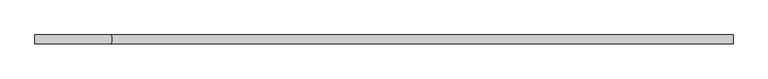
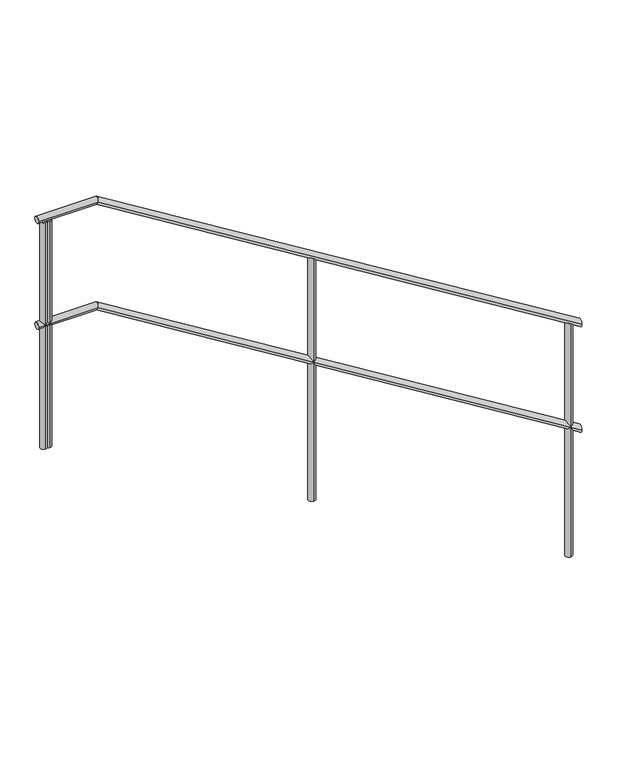
"""IFC4 building model written with IfcOpenShell, lengths in millimetres: railing geometry."""

from ifc_helpers import new_model, si_unit, point, frame, frame_2d, origin, place, context, project, spatial, circle_curve, ellipse_curve, trimmed, segment, composite_curve, outline, extrude, source, transform, mapped, element, save
from ifc_brep_helpers import plane_surface, cylinder_surface, advanced_brep


def railing_f185047e(model_context):
    return source(origin(), model_context, "Body", "SolidModel", [
        advanced_brep(
        [(68246.3017909, 71812.0208589, -450.9609787), (68246.3017909, 71842.0208589, -450.9609787), (66082.0450053, 71812.0208589, 885.0), (66082.0450053, 71842.0208589, 885.0), (65816.3017909, 71812.0208589, 885.0), (65816.3017909, 71842.0208589, 885.0)],
        [
            (0, 1, ellipse_curve(frame((68246.3017909, 71827.0208589, -450.9609787), z_axis=(1.0, 0.0, 0.0), x_axis=(0.0, 0.0, -1.0)), 17.6276454, 15.0)),
            (1, 0, ellipse_curve(frame((68246.3017909, 71827.0208589, -450.9609787), z_axis=(1.0, 0.0, 0.0), x_axis=(0.0, 0.0, -1.0)), 17.6276454, 15.0)),
            (0, 2),
            (2, 3, ellipse_curve(frame((66082.0450053, 71827.0208589, 885.0), z_axis=(0.9620125025549409, 0.0, -0.27300539358770864), x_axis=(-0.27300539358770803, 0.0, -0.9620125025549412)), 15.5923129, 15.0)),
            (3, 1),
            (3, 2, ellipse_curve(frame((66082.0450053, 71827.0208589, 885.0), z_axis=(0.9620125025549409, 0.0, -0.27300539358770864), x_axis=(-0.27300539358770803, 0.0, -0.9620125025549412)), 15.5923129, 15.0)),
            (4, 5, circle_curve(frame((65816.3017909, 71827.0208589, 885.0), z_axis=(-1.0, 0.0, 0.0), x_axis=(0.0, 1.0, 0.0)), 15.0)),
            (5, 4, circle_curve(frame((65816.3017909, 71827.0208589, 885.0), z_axis=(-1.0, 0.0, 0.0), x_axis=(0.0, 1.0, 0.0)), 15.0)),
            (2, 4),
            (5, 3),
        ],
        [
            plane_surface(frame((68246.3017909, 71827.0208589, -433.3333333), z_axis=(1.0, 0.0, 0.0), x_axis=(0.0, -1.0, 0.0))),
            cylinder_surface(frame((68238.4227528, 71827.0208589, -446.097375), z_axis=(0.8509361101440404, 0.0, -0.5252692037926168), x_axis=(0.0, 1.0, 0.0)), 15.0),
            plane_surface(frame((65816.3017909, 71827.0208589, 900.0), z_axis=(-1.0, 0.0, 0.0), x_axis=(0.0, -1.0, 0.0))),
            cylinder_surface(frame((66086.3017909, 71827.0208589, 885.0), z_axis=(1.0, 0.0, 0.0), x_axis=(0.0, 1.0, 0.0)), 15.0),
        ],
        [
            (0, [[1, 2]]),
            (1, [[-1, 3, 4, 5]]),
            (1, [[-2, -5, 6, -3]]),
            (2, [[7, 8]]),
            (3, [[-4, 9, -8, 10]]),
            (3, [[-6, -10, -7, -9]]),
        ],
    ),
        advanced_brep(
        [(68246.3017909, 71812.0208589, 49.0390213), (68246.3017909, 71842.0208589, 49.0390213), (66082.0450053, 71812.0208589, 1385.0), (66082.0450053, 71842.0208589, 1385.0), (65816.3017909, 71812.0208589, 1385.0), (65816.3017909, 71842.0208589, 1385.0)],
        [
            (0, 1, ellipse_curve(frame((68246.3017909, 71827.0208589, 49.0390213), z_axis=(1.0, 0.0, 0.0), x_axis=(0.0, 0.0, -1.0)), 17.6276454, 15.0)),
            (1, 0, ellipse_curve(frame((68246.3017909, 71827.0208589, 49.0390213), z_axis=(1.0, 0.0, 0.0), x_axis=(0.0, 0.0, -1.0)), 17.6276454, 15.0)),
            (0, 2),
            (2, 3, ellipse_curve(frame((66082.0450053, 71827.0208589, 1385.0), z_axis=(0.9620125025549409, 0.0, -0.27300539358770864), x_axis=(-0.27300539358770803, 0.0, -0.9620125025549412)), 15.5923129, 15.0)),
            (3, 1),
            (3, 2, ellipse_curve(frame((66082.0450053, 71827.0208589, 1385.0), z_axis=(0.9620125025549409, 0.0, -0.27300539358770864), x_axis=(-0.27300539358770803, 0.0, -0.9620125025549412)), 15.5923129, 15.0)),
            (4, 5, circle_curve(frame((65816.3017909, 71827.0208589, 1385.0), z_axis=(-1.0, 0.0, 0.0), x_axis=(0.0, 1.0, 0.0)), 15.0)),
            (5, 4, circle_curve(frame((65816.3017909, 71827.0208589, 1385.0), z_axis=(-1.0, 0.0, 0.0), x_axis=(0.0, 1.0, 0.0)), 15.0)),
            (2, 4),
            (5, 3),
        ],
        [
            plane_surface(frame((68246.3017909, 71827.0208589, 66.6666667), z_axis=(1.0, 0.0, 0.0), x_axis=(0.0, -1.0, 0.0))),
            cylinder_surface(frame((68238.4227528, 71827.0208589, 53.902625), z_axis=(0.8509361101440404, 0.0, -0.5252692037926168), x_axis=(0.0, 1.0, 0.0)), 15.0),
            plane_surface(frame((65816.3017909, 71827.0208589, 1400.0), z_axis=(-1.0, 0.0, 0.0), x_axis=(0.0, -1.0, 0.0))),
            cylinder_surface(frame((66086.3017909, 71827.0208589, 1385.0), z_axis=(1.0, 0.0, 0.0), x_axis=(0.0, 1.0, 0.0)), 15.0),
        ],
        [
            (0, [[1, 2]]),
            (1, [[-1, 3, 4, 5]]),
            (1, [[-2, -5, 6, -3]]),
            (2, [[7, 8]]),
            (3, [[-4, 9, -8, 10]]),
            (3, [[-6, -10, -7, -9]]),
        ],
    ),
        extrude(outline(composite_curve([segment(trimmed(circle_curve(frame_2d((65846.3017909, 71827.0208589)), 15.0), [point((65846.3017909, 71812.0208589))], [point((65846.3017909, 71842.0208589))], False, "CARTESIAN"), True, "CONTINUOUS"), segment(trimmed(circle_curve(frame_2d((65846.3017909, 71827.0208589)), 15.0), [point((65846.3017909, 71842.0208589))], [point((65846.3017909, 71812.0208589))], False, "CARTESIAN"), True, "CONTINUOUS")], self_intersect=False)), frame((0.0, 0.0, 300.0), z_axis=(0.0, 0.0, 1.0), x_axis=(1.0, 0.0, 0.0)), (0.0, 0.0, 1.0), 1070.0),
        advanced_brep(
        [(67046.3017909, 71842.0208589, 777.4074074), (67046.3017909, 71842.0208589, -366.6666667), (67046.3017909, 71812.0208589, -366.6666667), (67046.3017909, 71812.0208589, 777.4074074)],
        [
            (0, 1),
            (1, 2, circle_curve(frame((67046.3017909, 71827.0208589, -366.6666667), z_axis=(0.0, 0.0, 1.0), x_axis=(0.0, -1.0, 0.0)), 15.0)),
            (2, 3),
            (3, 0, ellipse_curve(frame((67046.3017909, 71827.0208589, 777.4074074), z_axis=(-0.5252692037926167, 0.0, -0.8509361101440406), x_axis=(-0.8509361101440406, 0.0, 0.5252692037926162)), 17.6276454, 15.0)),
            (0, 3, ellipse_curve(frame((67046.3017909, 71827.0208589, 777.4074074), z_axis=(-0.5252692037926167, 0.0, -0.8509361101440406), x_axis=(-0.8509361101440406, 0.0, 0.5252692037926162)), 17.6276454, 15.0)),
            (2, 1, circle_curve(frame((67046.3017909, 71827.0208589, -366.6666667), z_axis=(0.0, 0.0, 1.0), x_axis=(0.0, -1.0, 0.0)), 15.0)),
        ],
        [
            cylinder_surface(frame((67046.3017909, 71827.0208589, -466.6666667), z_axis=(0.0, 0.0, 1.0), x_axis=(0.0, -1.0, 0.0)), 15.0),
            plane_surface(frame((67021.3017909, 71802.0208589, 792.8395062), z_axis=(0.5252692037926167, 0.0, 0.8509361101440406), x_axis=(0.0, 1.0, 0.0))),
            plane_surface(frame((67071.3017909, 71802.0208589, -366.6666667), z_axis=(0.0, 0.0, -1.0), x_axis=(0.0, 1.0, 0.0))),
        ],
        [
            (0, [[1, 2, 3, 4]]),
            (0, [[-1, 5, -3, 6]]),
            (1, [[-4, -5]]),
            (2, [[-2, -6]]),
        ],
    ),
        extrude(outline(composite_curve([segment(trimmed(circle_curve(frame_2d((65866.3017909, 71827.0208589)), 15.0), [point((65866.3017909, 71812.0208589))], [point((65866.3017909, 71842.0208589))], False, "CARTESIAN"), True, "CONTINUOUS"), segment(trimmed(circle_curve(frame_2d((65866.3017909, 71827.0208589)), 15.0), [point((65866.3017909, 71842.0208589))], [point((65866.3017909, 71812.0208589))], False, "CARTESIAN"), True, "CONTINUOUS")], self_intersect=False)), frame((0.0, 0.0, 300.0), z_axis=(0.0, 0.0, 1.0), x_axis=(1.0, 0.0, 0.0)), (0.0, 0.0, 1.0), 1070.0),
        advanced_brep(
        [(68196.3017909, 71842.0208589, 67.5308642), (68196.3017909, 71842.0208589, -1033.3333333), (68196.3017909, 71812.0208589, -1033.3333333), (68196.3017909, 71812.0208589, 67.5308642)],
        [
            (0, 1),
            (1, 2, circle_curve(frame((68196.3017909, 71827.0208589, -1033.3333333), z_axis=(0.0, 0.0, 1.0), x_axis=(0.0, -1.0, 0.0)), 15.0)),
            (2, 3),
            (3, 0, ellipse_curve(frame((68196.3017909, 71827.0208589, 67.5308642), z_axis=(-0.5252692037926167, 0.0, -0.8509361101440406), x_axis=(-0.8509361101440406, 0.0, 0.5252692037926162)), 17.6276454, 15.0)),
            (0, 3, ellipse_curve(frame((68196.3017909, 71827.0208589, 67.5308642), z_axis=(-0.5252692037926167, 0.0, -0.8509361101440406), x_axis=(-0.8509361101440406, 0.0, 0.5252692037926162)), 17.6276454, 15.0)),
            (2, 1, circle_curve(frame((68196.3017909, 71827.0208589, -1033.3333333), z_axis=(0.0, 0.0, 1.0), x_axis=(0.0, -1.0, 0.0)), 15.0)),
        ],
        [
            cylinder_surface(frame((68196.3017909, 71827.0208589, -1133.3333333), z_axis=(0.0, 0.0, 1.0), x_axis=(0.0, -1.0, 0.0)), 15.0),
            plane_surface(frame((68171.3017909, 71802.0208589, 82.962963), z_axis=(0.5252692037926167, 0.0, 0.8509361101440406), x_axis=(0.0, 1.0, 0.0))),
            plane_surface(frame((68221.3017909, 71802.0208589, -1033.3333333), z_axis=(0.0, 0.0, -1.0), x_axis=(0.0, 1.0, 0.0))),
        ],
        [
            (0, [[1, 2, 3, 4]]),
            (0, [[-1, 5, -3, 6]]),
            (1, [[-4, -5]]),
            (2, [[-2, -6]]),
        ],
    ),
    ])


if __name__ == "__main__":
    model = new_model("IFC4")
    model_context = context("Model", 3, world=origin())
    ifc_project = project(units=[si_unit("LENGTHUNIT", "METRE", prefix="MILLI")], contexts=[model_context])
    site = spatial("IfcSite", under=ifc_project)
    building = spatial("IfcBuilding", under=site)
    placement = place(None, origin())
    railing_shape = railing_f185047e(model_context)
    element("IfcRailing", 1, at=placement, inside=building, context=model_context, shape_type="MappedRepresentation", body=[
        mapped(railing_shape, transform((0.0, 0.0, 0.0), x_axis=(1.0, 0.0, 0.0), y_axis=(0.0, 1.0, 0.0), z_axis=(0.0, 0.0, 1.0))),
    ])
    save(model, "model.ifc")
